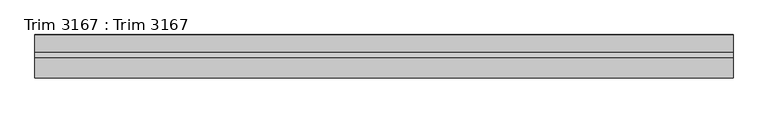
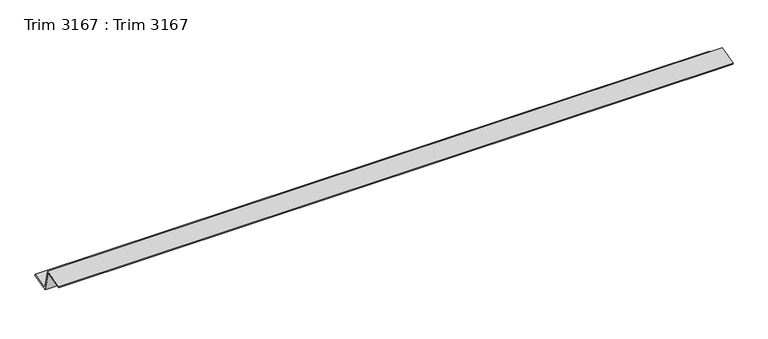
"""IFC4 building model written with IfcOpenShell, lengths in millimetres: proxy geometry, Trim 3167 : Trim 3167."""

from ifc_helpers import new_model, si_unit, frame, origin, place, context, project, spatial, polyline, outline, extrude, source, transform, mapped, element, save


def trim_3167_trim_3167_1625afa1(model_context):
    return source(origin(), model_context, "Body", "SweptSolid", [
        extrude(outline(polyline([(10630.9111328, 43879.0351562), (10613.78125, 43941.7109375), (10560.7460937, 43928.2890625), (10559.7647325, 43932.1668106), (10616.6049434, 43946.55165), (10633.7356926, 43883.8726984), (10682.5824336, 43896.1910686), (10683.5605469, 43892.3125), (10630.9111328, 43879.0351562)])), frame((3694.2883192, 0.0, 0.0), z_axis=(1.0, 0.0, 0.0), x_axis=(0.0, 1.0, 0.0)), (0.0, 0.0, 1.0), 2000.0),
    ])


if __name__ == "__main__":
    model = new_model("IFC4")
    model_context = context("Model", 3, world=origin())
    ifc_project = project(units=[si_unit("LENGTHUNIT", "METRE", prefix="MILLI")], contexts=[model_context])
    site = spatial("IfcSite", under=ifc_project)
    building = spatial("IfcBuilding", under=site)
    placement = place(None, origin())
    trim_3167_trim_3167_shape = trim_3167_trim_3167_1625afa1(model_context)
    element("IfcBuildingElementProxy", 1, Name="Trim 3167 : Trim 3167", ObjectType="Trim 3167 : Trim 3167", at=placement, inside=building, context=model_context, shape_type="MappedRepresentation", body=[
        mapped(trim_3167_trim_3167_shape, transform((0.0, 0.0, 0.0), x_axis=(1.0, 0.0, 0.0), y_axis=(0.0, 1.0, 0.0), z_axis=(0.0, 0.0, 1.0))),
    ])
    save(model, "model.ifc")

# Revit data of these elements
# Type "Trim 3167 : Trim 3167"
#   NameOverride = "Trim"
# Element 1 (IfcBuildingElementProxy, "Trim 3167 : Trim 3167")
#   Materials on its faces: "ZEE CLOSURE TRIM"
# Materials
#   "ZEE CLOSURE TRIM": class "Unassigned", colour RGB 128 128 128, transparency 0
